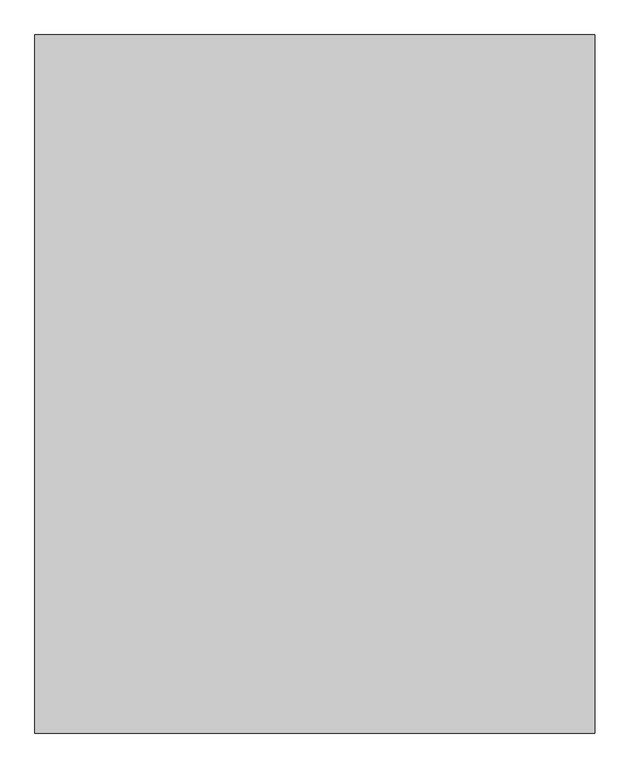
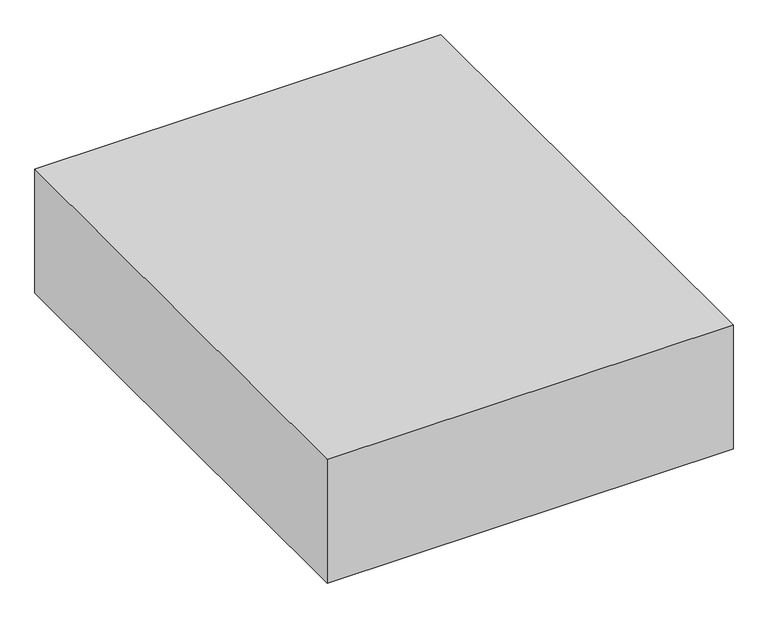
"""IFC4 building model written with IfcOpenShell, lengths in millimetres: proxy geometry, Space Planning Box_hec : Space Planning Box_hec."""

from ifc_helpers import new_model, si_unit, origin, origin_with_axes, place, context, project, spatial, polyline, outline, extrude, source, transform, mapped, element, save


def generic_models_d82b1902(model_context):
    return source(origin(), model_context, "Body", "SweptSolid", [
        extrude(outline(polyline([(9300.0, 11600.0), (9300.0, -11600.0), (-9300.0, -11600.0), (-9300.0, 11600.0), (9300.0, 11600.0)])), origin_with_axes(), (0.0, 0.0, 1.0), 6000.0),
    ])


if __name__ == "__main__":
    model = new_model("IFC4")
    model_context = context("Model", 3, world=origin())
    ifc_project = project(units=[si_unit("LENGTHUNIT", "METRE", prefix="MILLI")], contexts=[model_context])
    site = spatial("IfcSite", under=ifc_project)
    building = spatial("IfcBuilding", under=site)
    placement = place(None, origin())
    generic_models_shape = generic_models_d82b1902(model_context)
    element("IfcBuildingElementProxy", 1, Name="Space Planning Box_hec : Space Planning Box_hec", ObjectType="Space Planning Box_hec : Space Planning Box_hec", at=placement, inside=building, context=model_context, shape_type="MappedRepresentation", body=[
        mapped(generic_models_shape, transform((0.0, 0.0, 0.0), x_axis=(1.0, 0.0, 0.0), y_axis=(0.0, 1.0, 0.0), z_axis=(0.0, 0.0, 1.0))),
    ])
    save(model, "model.ifc")

# Revit data of these elements
# Type "Space Planning Box_hec : Space Planning Box_hec"
#   Type Comments = "..."
#   Room Name [instance default] = "?"
#   Interior Finish [instance default] = ""
#   Exterior Finish [instance default] = ""
#   Department [instance default] = ""
#   Assembly Code = "..."
#   Width [instance default] = 1524 mm
#   Program Area [instance default] = 0 m²
#   Length [instance default] = 1524 mm
#   Height [instance default] = 1524 mm
#   Area [instance default] = 2.32258 m²
#   Fill Color [instance default] = Cyan
#   Default Elevation = 0
# Element 1 (IfcBuildingElementProxy, "Space Planning Box_hec : Space Planning Box_hec")
#   Room Name = "Electronic Room"
#   Interior Finish = "IF1"
#   Exterior Finish = "EF1"
#   Department = "CI"
#   Width = 18600 mm
#   Program Area = 431.52 m²
#   Length = 23200 mm
#   Height = 6000 mm
#   Area = 431.52 m²
#   Fill Color = Lime
#   Materials on its faces: "Lime"
# Materials
#   "Cyan": class "Generic", colour RGB 0 255 255, transparency 0.2, Cost = 0
#   "Lime": class "Generic", colour RGB 0 255 0, transparency 0.2, Cost = 0
